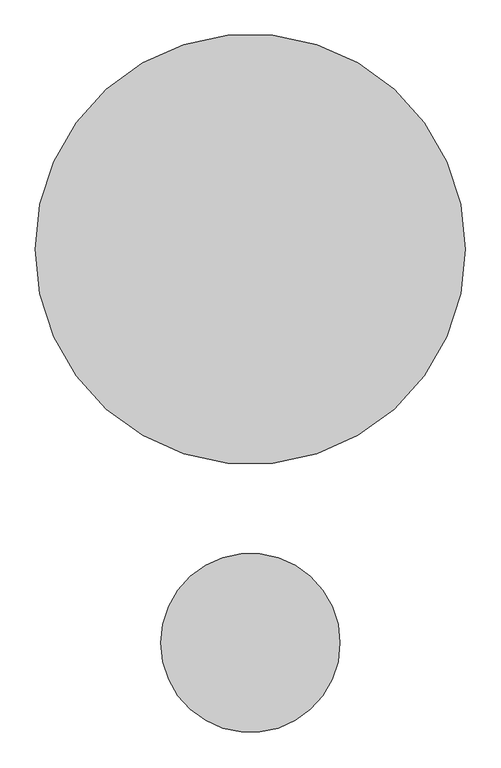
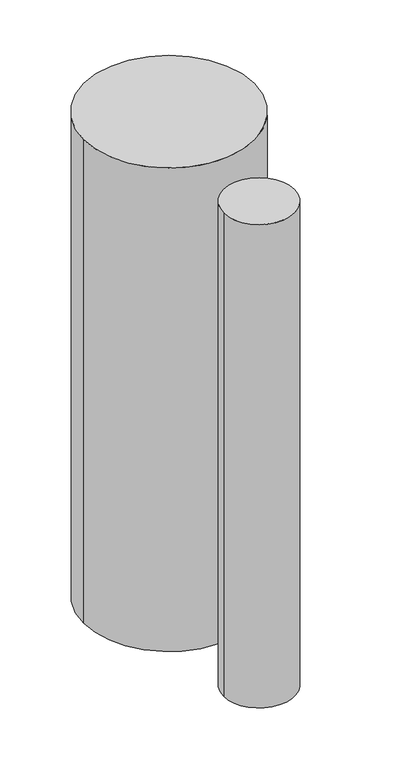
"""IFC4 building model written with IfcOpenShell, lengths in millimetres: proxy geometry, GENERIC WATER SOFTENER & BRINE TANK : GENERIC WATER SOFTENER & BRINE TANK."""

from ifc_helpers import new_model, si_unit, point, frame_2d, origin, origin_with_axes, origin_2d, place, context, project, spatial, circle_curve, trimmed, segment, composite_curve, outline, extrude, source, transform, mapped, element, save


def mechanical_equipment_c073f697(model_context):
    return source(origin(), model_context, "Body", "SweptSolid", [
        extrude(outline(composite_curve([segment(trimmed(circle_curve(origin_2d(), 127.0), [point((-127.0, 0.0))], [point((127.0, 0.0))], False, "CARTESIAN"), True, "CONTINUOUS"), segment(trimmed(circle_curve(origin_2d(), 127.0), [point((127.0, 0.0))], [point((-127.0, 0.0))], False, "CARTESIAN"), True, "CONTINUOUS")], self_intersect=False)), origin_with_axes(), (0.0, 0.0, 1.0), 1828.8),
        extrude(outline(composite_curve([segment(trimmed(circle_curve(frame_2d((0.0, 557.8519486)), 304.8), [point((-304.8, 557.8519486))], [point((304.8, 557.8519486))], False, "CARTESIAN"), True, "CONTINUOUS"), segment(trimmed(circle_curve(frame_2d((0.0, 557.8519486)), 304.8), [point((304.8, 557.8519486))], [point((-304.8, 557.8519486))], False, "CARTESIAN"), True, "CONTINUOUS")], self_intersect=False)), origin_with_axes(), (0.0, 0.0, 1.0), 1828.8),
    ])


if __name__ == "__main__":
    model = new_model("IFC4")
    model_context = context("Model", 3, world=origin())
    ifc_project = project(units=[si_unit("LENGTHUNIT", "METRE", prefix="MILLI")], contexts=[model_context])
    site = spatial("IfcSite", under=ifc_project)
    building = spatial("IfcBuilding", under=site)
    placement = place(None, origin())
    mechanical_equipment_shape = mechanical_equipment_c073f697(model_context)
    element("IfcBuildingElementProxy", 1, Name="GENERIC WATER SOFTENER & BRINE TANK : GENERIC WATER SOFTENER & BRINE TANK", ObjectType="GENERIC WATER SOFTENER & BRINE TANK : GENERIC WATER SOFTENER & BRINE TANK", at=placement, inside=building, context=model_context, shape_type="MappedRepresentation", body=[
        mapped(mechanical_equipment_shape, transform((0.0, 0.0, 0.0), x_axis=(1.0, 0.0, 0.0), y_axis=(0.0, 1.0, 0.0), z_axis=(0.0, 0.0, 1.0))),
    ])
    save(model, "model.ifc")
